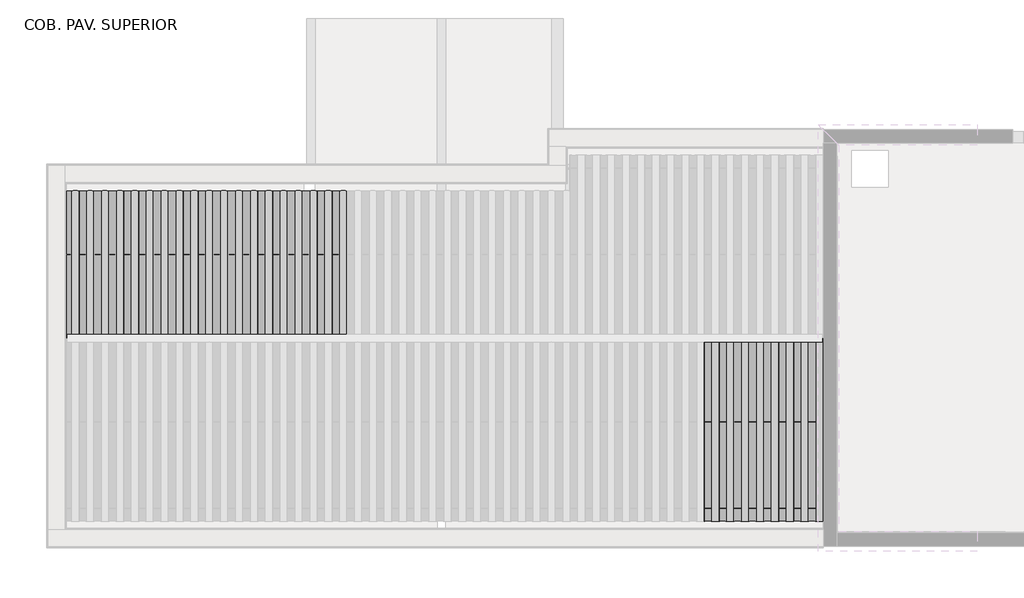
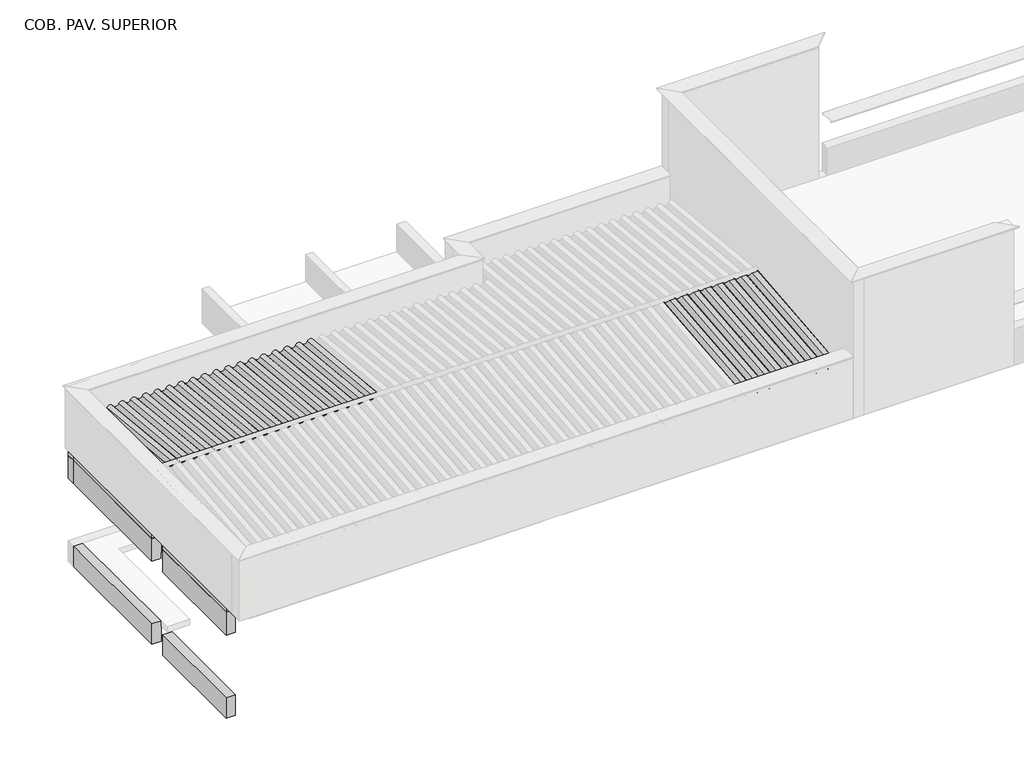
# One storey, part 3 of 7: 39 beams, 5 columns.
# Revit data of these elements (continued)
# Type "Madeira de lei : Berço 6x12cm"
#   A = 0.02 m²
#   Length [instance default] = 1.524 m
#   b = 0.06 m
#   d = 0.12 m
#   Structural Material [instance default] = none
#   Assembly Code = ""
# Type "TQS - Viga retangular : 19.0 x 45.0"
#   Length [instance default] = 1.524 m
#   b = 0.19 m
#   h = 0.45 m
#   Structural Material [instance default] = none
#   Assembly Code = ""
# Type "TQS - Viga retangular : 19.0 x 50.0"
#   Length [instance default] = 1.524 m
#   b = 0.19 m
#   h = 0.50 m
#   Structural Material [instance default] = none
#   Assembly Code = ""
# Type "TQS - Viga retangular : 19.0 x 90.0"
#   Length [instance default] = 1.524 m
#   b = 0.19 m
#   h = 0.90 m
#   Structural Material [instance default] = none
#   Assembly Code = ""
# Type "Telha Ondulada : Fibrocimento"
#   Description = "TELHA ONDULADA FIBROCIMENTO"
#   Cost = 5
#   Length [instance default] = 1.524 m
#   b = 0.07 m
#   h = 0.16 m
#   Structural Material = .TELHA DE FIBROCIMENTO
#   Assembly Code = ""
# Type "Madeira de lei-Coluna : Pontalete 6X16cm"
#   A = 0.01952 m²
#   b = 0.06 m
#   d = 0.16 m
#   Structural Material [instance default] = none
#   Assembly Code = ""
# Elements 1, 2, 3, 4, 5, 6, 7 (IfcBeam, "Madeira de lei : Berço 6x12cm")
#   Comments = ""
#   Structural Material = .MADEIRAMENTO
#   Phase Created = CC_PE
#   Materials on its faces: ".MADEIRAMENTO"
# Element 8 (IfcBeam, "TQS - Viga retangular : 19.0 x 45.0")
#   Uso = "ESTRUTURA"
#   Titulo = "V412"
#   Chave = "-487"
#   Tipo Elemento = "Viga"
#   SHA1 = "0B82E8DE04504795958F5A57F4D5042EC674D83A"
#   Revisão = ""
#   Tipo de carga = ""
#   Divisor de flexao = ""
#   Secao = ""
#   Configuracao = ""
#   Angulo (graus) = ""
#   Detalhamento = ""
#   Casos de vento manual = ""
#   Tipo = ""
#   Alcas = ""
#   Furos = ""
#   Pino = ""
#   Distribuicao = ""
#   Solidarizado = ""
#   Solidarizar na montagem = ""
#   Unir com o próximo = ""
#   Grupo pre moldado = ""
#   Verificado = ""
#   Concreto C = ""
#   Taxa de armadura (kgf/m³) = 0
#   Carga (tf/m²) = 0
#   Carga (tf/m) = 0
#   Carga (tf) = 0
#   Altura = 0.45 m
#   Rebaixo = 0.00 m
#   Largura = 0.19 m
#   Distancia a face = 0.00 m
#   Distancia ao eixo = 0.00 m
#   Altura gerber esquerda = 0.00 m
#   Largura gerber esquerda = 0.00 m
#   Altura gerber direita = 0.00 m
#   Largura gerber direita = 0.00 m
#   Resultado de Ensaios fck (MPa) = 0
#   Unique TQS ID = -487
#   Principal = yes
#   Structural Material = none
#   Phase Created = CC_PE
# Element 9 (IfcBeam, "TQS - Viga retangular : 19.0 x 50.0")
#   Uso = "ESTRUTURA"
#   Titulo = "V405"
#   Chave = "-481"
#   Tipo Elemento = "Viga"
#   SHA1 = "62B8C69EE67CDAF062D98DEB998082D18D2F4D4C"
#   Revisão = ""
#   Tipo de carga = ""
#   Divisor de flexao = ""
#   Secao = ""
#   Configuracao = ""
#   Angulo (graus) = ""
#   Detalhamento = ""
#   Casos de vento manual = ""
#   Tipo = ""
#   Alcas = ""
#   Furos = ""
#   Pino = ""
#   Distribuicao = ""
#   Solidarizado = ""
#   Solidarizar na montagem = ""
#   Unir com o próximo = ""
#   Grupo pre moldado = ""
#   Verificado = ""
#   Concreto C = ""
#   Taxa de armadura (kgf/m³) = 0
#   Carga (tf/m²) = 0
#   Carga (tf/m) = 0
#   Carga (tf) = 0
#   Altura = 0.50 m
#   Rebaixo = -0.50 m
#   Largura = 0.19 m
#   Distancia a face = 0.00 m
#   Distancia ao eixo = 0.00 m
#   Altura gerber esquerda = 0.00 m
#   Largura gerber esquerda = 0.00 m
#   Altura gerber direita = 0.00 m
#   Largura gerber direita = 0.00 m
#   Resultado de Ensaios fck (MPa) = 0
#   Unique TQS ID = -481
#   Principal = yes
#   Structural Material = none
#   Phase Created = CC_PE
# Element 10 (IfcBeam, "TQS - Viga retangular : 19.0 x 50.0")
#   Uso = "ESTRUTURA"
#   Titulo = "V413"
#   Chave = "-479"
#   Tipo Elemento = "Viga"
#   SHA1 = "0050BE578970BB6D063616F79CD9D0E5B8A688B2"
#   Revisão = ""
#   Tipo de carga = ""
#   Divisor de flexao = ""
#   Secao = ""
#   Configuracao = ""
#   Angulo (graus) = ""
#   Detalhamento = ""
#   Casos de vento manual = ""
#   Tipo = ""
#   Alcas = ""
#   Furos = ""
#   Pino = ""
#   Distribuicao = ""
#   Solidarizado = ""
#   Solidarizar na montagem = ""
#   Unir com o próximo = ""
#   Grupo pre moldado = ""
#   Verificado = ""
#   Concreto C = ""
#   Taxa de armadura (kgf/m³) = 0
#   Carga (tf/m²) = 0
#   Carga (tf/m) = 0
#   Carga (tf) = 0
#   Altura = 0.50 m
#   Rebaixo = -0.50 m
#   Largura = 0.19 m
#   Distancia a face = 0.00 m
#   Distancia ao eixo = 0.00 m
#   Altura gerber esquerda = 0.00 m
#   Largura gerber esquerda = 0.00 m
#   Altura gerber direita = 0.00 m
#   Largura gerber direita = 0.00 m
#   Resultado de Ensaios fck (MPa) = 0
#   Unique TQS ID = -479
#   Principal = yes
#   Structural Material = none
#   Phase Created = CC_PE
# Element 11 (IfcBeam, "TQS - Viga retangular : 19.0 x 90.0")
#   Uso = "ESTRUTURA"
#   Titulo = "V404"
#   Chave = "-413"
#   Tipo Elemento = "Viga"
#   SHA1 = "523F9EBFA0808C71AB4CE075FF02A0A51CF03D70"
#   Revisão = ""
#   Tipo de carga = ""
#   Divisor de flexao = ""
#   Secao = ""
#   Configuracao = ""
#   Angulo (graus) = ""
#   Detalhamento = ""
#   Casos de vento manual = ""
#   Tipo = ""
#   Alcas = ""
#   Furos = ""
#   Pino = ""
#   Distribuicao = ""
#   Solidarizado = ""
#   Solidarizar na montagem = ""
#   Unir com o próximo = ""
#   Grupo pre moldado = ""
#   Verificado = ""
#   Concreto C = ""
#   Taxa de armadura (kgf/m³) = 0
#   Carga (tf/m²) = 0
#   Carga (tf/m) = 0
#   Carga (tf) = 0
#   Altura = 0.90 m
#   Rebaixo = -0.6105 m
#   Largura = 0.19 m
#   Distancia a face = 0.00 m
#   Distancia ao eixo = 0.00 m
#   Altura gerber esquerda = 0.00 m
#   Largura gerber esquerda = 0.00 m
#   Altura gerber direita = 0.00 m
#   Largura gerber direita = 0.00 m
#   Resultado de Ensaios fck (MPa) = 0
#   Unique TQS ID = -413
#   Principal = yes
#   Structural Material = none
#   Phase Created = CC_PE
# Element 12 (IfcBeam, "TQS - Viga retangular : 19.0 x 90.0")
#   Uso = "ESTRUTURA"
#   Titulo = "V414"
#   Chave = "-404"
#   Tipo Elemento = "Viga"
#   SHA1 = "CE060170271A1EAF38D9C4F52A5150784927B7FC"
#   Revisão = ""
#   Tipo de carga = ""
#   Divisor de flexao = ""
#   Secao = ""
#   Configuracao = ""
#   Angulo (graus) = ""
#   Detalhamento = ""
#   Casos de vento manual = ""
#   Tipo = ""
#   Alcas = ""
#   Furos = ""
#   Pino = ""
#   Distribuicao = ""
#   Solidarizado = ""
#   Solidarizar na montagem = ""
#   Unir com o próximo = ""
#   Grupo pre moldado = ""
#   Verificado = ""
#   Concreto C = ""
#   Taxa de armadura (kgf/m³) = 0
#   Carga (tf/m²) = 0
#   Carga (tf/m) = 0
#   Carga (tf) = 0
#   Altura = 0.90 m
#   Rebaixo = -0.6105 m
#   Largura = 0.19 m
#   Distancia a face = 0.00 m
#   Distancia ao eixo = 0.00 m
#   Altura gerber esquerda = 0.00 m
#   Largura gerber esquerda = 0.00 m
#   Altura gerber direita = 0.00 m
#   Largura gerber direita = 0.00 m
#   Resultado de Ensaios fck (MPa) = 0
#   Unique TQS ID = -404
#   Principal = yes
#   Structural Material = none
#   Phase Created = CC_PE
# Elements 13, 14, 15, 16, 17, 18, 19, 20, 21, 22, 23, 24, 25, 26, 27, 28, 29, 30, 31, 32, 33, 34, 35, 36, 37, 38, 39 (IfcBeam, "Telha Ondulada : Fibrocimento")
#   Phase Created = CC_PE
#   Materials on its faces: ".TELHA DE FIBROCIMENTO"
# Elements 40, 41, 42, 43, 44 (IfcColumn, "Madeira de lei-Coluna : Pontalete 6X16cm")
#   Comments = ""
#   Structural Material = .MADEIRAMENTO
#   Phase Created = CC_PE
#   Materials on its faces: ".MADEIRAMENTO"
# Materials
#   ".TELHA DE FIBROCIMENTO": class "CC_TELHADO", colour RGB 77 77 76, transparency 0, Description = "TELHA ONDULADA FIBROCIMENTO", Cost = 0
#   ".MADEIRAMENTO": class ".CC_MADEIRAS", colour RGB 212 179 113, transparency 0, Cost = 0
